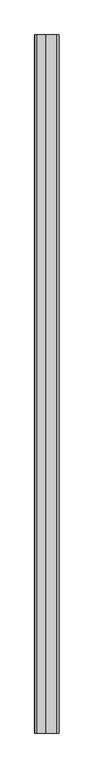
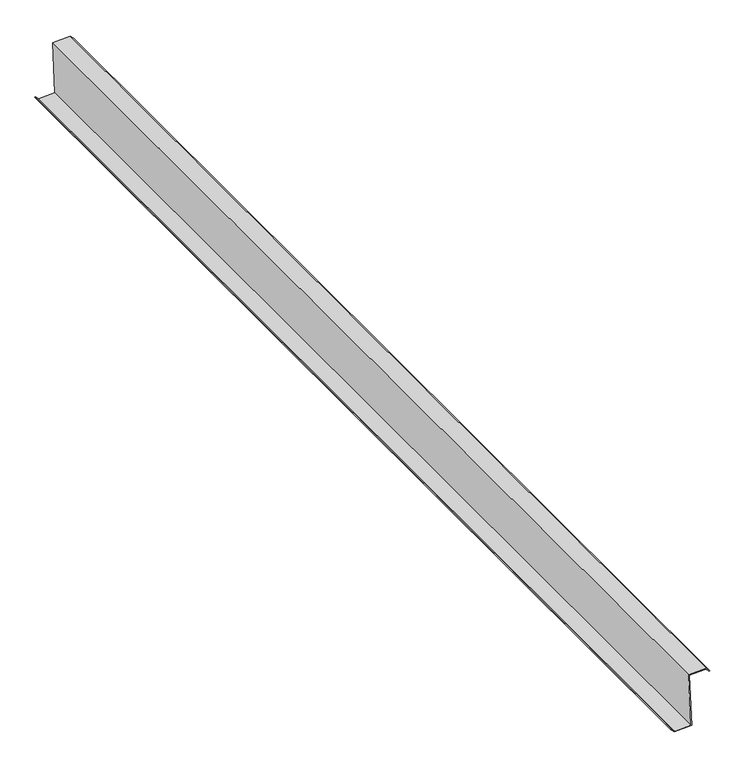
"""IFC4 building model written with IfcOpenShell, lengths in millimetres: proxy geometry, Generic Models 7:Generic Models 1:337419:Generic Models 1:337419 : Generic Models 7:Generic Models 1:337419:3 : Generic Models 7:Generic Models 1:337419:Generic Models 1:337419 : Generic Models 7:Generic Models 1:337419:301336."""

import ifcopenshell
import ifcopenshell.guid

model = None  # the IFC model being written
_history = None  # IfcOwnerHistory: only IFC2X3 demands one
_inside = {}  # id of a spatial element -> (the spatial element, [elements in it])
_under = {}  # id of a project, library or spatial element -> (it, [spatial elements below it])
_declared = {}  # id of a project -> (the project, [libraries it declares])
_typed = {}  # id of a type object -> (the type object, [elements of that type])
_made_of = {}  # id of a material, layer set ... -> (it, [elements and type objects made of it])


def new_model(schema):
    """Start an empty IFC model of exactly this schema.

    Asked for "IFC4X3", IfcOpenShell would pick the latest addendum, in which some entities
    have other attributes; the version numbers below select the first issue.
    IFC2X3 requires an IfcOwnerHistory on every rooted entity: one is made here for all.
    """
    global model, _history
    if schema == "IFC4X3":
        model = ifcopenshell.file(schema_version=(4, 3, 0, 0))
    else:
        model = ifcopenshell.file(schema=schema)
    _inside.clear()
    _under.clear()
    _declared.clear()
    _typed.clear()
    _made_of.clear()
    _history = None
    if model.schema == "IFC2X3":
        org = make("IfcOrganization", Name="unknown")
        user = make(
            "IfcPersonAndOrganization",
            ThePerson=make("IfcPerson", FamilyName="unknown"),
            TheOrganization=org,
        )
        app = make(
            "IfcApplication",
            ApplicationDeveloper=org,
            Version="unknown",
            ApplicationFullName="unknown",
            ApplicationIdentifier="unknown",
        )
        _history = make(
            "IfcOwnerHistory",
            OwningUser=user,
            OwningApplication=app,
            ChangeAction="ADDED",
            CreationDate=0,
        )
    return model


def make(cls, **values):
    """One entity of the class cls with the attributes given. An attribute that is None is left unset."""
    return model.create_entity(
        cls, **{name: value for name, value in values.items() if value is not None}
    )


def rooted(cls, **values):
    """An entity with a GlobalId (a new one), such as an element, a storey or a relation."""
    return make(cls, GlobalId=ifcopenshell.guid.new(), OwnerHistory=_history, **values)


def si_unit(unit_type, name, prefix=None):
    """IfcSIUnit, for example si_unit("LENGTHUNIT", "METRE", prefix="MILLI")."""
    return make("IfcSIUnit", UnitType=unit_type, Prefix=prefix, Name=name)


def assignment(units):
    """IfcUnitAssignment: the units of a project."""
    return None if units is None else make("IfcUnitAssignment", Units=units)


def point(xyz):
    """IfcCartesianPoint."""
    return None if xyz is None else make("IfcCartesianPoint", Coordinates=xyz)


def direction(xyz):
    """IfcDirection."""
    return None if xyz is None else make("IfcDirection", DirectionRatios=xyz)


def frame(location, z_axis=None, x_axis=None):
    """IfcAxis2Placement3D, a coordinate frame: its origin and axes. An axis left out is left unset."""
    return make(
        "IfcAxis2Placement3D",
        Location=point(location),
        Axis=direction(z_axis),
        RefDirection=direction(x_axis),
    )


def origin():
    """The frame at (0, 0, 0) with its axes left unset."""
    return frame((0.0, 0.0, 0.0))


def place(relative_to, where):
    """IfcLocalPlacement: puts the frame where relative to a parent placement (None: the world)."""
    return make(
        "IfcLocalPlacement", PlacementRelTo=relative_to, RelativePlacement=where
    )


def context(
    kind, dimensions, precision=None, world=None, true_north=None, identifier=None
):
    """IfcGeometricRepresentationContext, for example the 3D "Model" context."""
    return make(
        "IfcGeometricRepresentationContext",
        ContextIdentifier=identifier,
        ContextType=kind,
        CoordinateSpaceDimension=dimensions,
        Precision=precision,
        WorldCoordinateSystem=world,
        TrueNorth=true_north,
    )


def project(units=None, contexts=None):
    """IfcProject with its units and contexts."""
    return rooted(
        "IfcProject",
        Name="project",
        RepresentationContexts=contexts,
        UnitsInContext=assignment(units),
    )


def spatial(cls, under=None, at=None, **own):
    """A site, building, storey or space (cls), placed at a placement, below another one or the project."""
    s = rooted(cls, ObjectPlacement=at, **own)
    if under is not None:
        _under.setdefault(under.id(), (under, []))[1].append(s)
    return s


def polyline(points):
    """IfcPolyline through the points."""
    return make("IfcPolyline", Points=[point(p) for p in points])


def outline(outer, holes=None, kind="AREA"):
    """IfcArbitraryClosedProfileDef: a profile drawn as a closed curve; with holes, ...WithVoids."""
    if holes is None:
        return make("IfcArbitraryClosedProfileDef", ProfileType=kind, OuterCurve=outer)
    return make(
        "IfcArbitraryProfileDefWithVoids",
        ProfileType=kind,
        OuterCurve=outer,
        InnerCurves=holes,
    )


def extrude(swept, where, along, depth):
    """IfcExtrudedAreaSolid: the profile swept, set in the frame where, extruded along a direction by depth."""
    return make(
        "IfcExtrudedAreaSolid",
        SweptArea=swept,
        Position=where,
        ExtrudedDirection=direction(along),
        Depth=depth,
    )


def shape(context_of_items, identifier, shape_type, items):
    """IfcShapeRepresentation: the items that make up one representation, for example the "Body"."""
    return make(
        "IfcShapeRepresentation",
        ContextOfItems=context_of_items,
        RepresentationIdentifier=identifier,
        RepresentationType=shape_type,
        Items=items,
    )


def source(mapping_origin, context_of_items, identifier, shape_type, items):
    """IfcRepresentationMap: a shape defined once, which mapped items show again and again."""
    return make(
        "IfcRepresentationMap",
        MappingOrigin=mapping_origin,
        MappedRepresentation=shape(context_of_items, identifier, shape_type, items),
    )


def transform(
    local_origin,
    x_axis=None,
    y_axis=None,
    z_axis=None,
    scale=None,
    scale2=None,
    scale3=None,
    uniform=True,
):
    """IfcCartesianTransformationOperator3D, or its non-uniform kind. x_axis, y_axis, z_axis: its Axis1, 2, 3."""
    if uniform:
        return make(
            "IfcCartesianTransformationOperator3D",
            Axis1=direction(x_axis),
            Axis2=direction(y_axis),
            LocalOrigin=point(local_origin),
            Scale=scale,
            Axis3=direction(z_axis),
        )
    return make(
        "IfcCartesianTransformationOperator3DnonUniform",
        Axis1=direction(x_axis),
        Axis2=direction(y_axis),
        LocalOrigin=point(local_origin),
        Scale=scale,
        Axis3=direction(z_axis),
        Scale2=scale2,
        Scale3=scale3,
    )


def mapped(mapping_source, mapping_target):
    """IfcMappedItem: shows the shape of a source again, moved by a transform."""
    return make(
        "IfcMappedItem", MappingSource=mapping_source, MappingTarget=mapping_target
    )


def made_of(thing, what):
    """Note that an element or type object is made of a material, layer set ...; save() writes the relation."""
    if what is not None:
        _made_of.setdefault(what.id(), (what, []))[1].append(thing)
    return thing


def element(
    cls,
    number,
    at=None,
    inside=None,
    cuts=None,
    type_object=None,
    material=None,
    context=None,
    identifier="Body",
    shape_type=None,
    held_by="IfcProductDefinitionShape",
    body=None,
    shapes=None,
    **own,
):
    """One element of the class cls, such as IfcWall. Its Tag is "e" and its number.

    at: its placement. inside: the storey or other place that contains it. cuts: it is an
    opening in that element (IfcRelVoidsElement). A single representation is given by context,
    identifier, shape_type and body (its items); several are given by shapes. held_by: the class
    of the entity that holds the representations. save() writes the other relations.
    """
    e = rooted(cls, Tag="e%d" % number, ObjectPlacement=at, **own)
    if body is not None:
        shapes = [shape(context, identifier, shape_type, body)]
    if shapes is not None:
        e.Representation = make(held_by, Representations=shapes)
    if inside is not None:
        _inside.setdefault(inside.id(), (inside, []))[1].append(e)
    if cuts is not None:
        rooted(
            "IfcRelVoidsElement", RelatingBuildingElement=cuts, RelatedOpeningElement=e
        )
    if type_object is not None:
        _typed.setdefault(type_object.id(), (type_object, []))[1].append(e)
    return made_of(e, material)


def aggregate(whole, parts):
    """IfcRelAggregates: a whole, such as a stair, and the parts it consists of."""
    return rooted("IfcRelAggregates", RelatingObject=whole, RelatedObjects=parts)


def save(model, path):
    """Write the relations noted so far, then the file.

    IfcRelAggregates (storeys below a building ...), IfcRelContainedInSpatialStructure (elements
    in a storey), IfcRelDefinesByType, IfcRelAssociatesMaterial and IfcRelDeclares: one each for
    every whole, place, type object, material and project.
    """
    for whole, parts in _under.values():
        aggregate(whole, parts)
    for where, things in _inside.values():
        rooted(
            "IfcRelContainedInSpatialStructure",
            RelatedElements=things,
            RelatingStructure=where,
        )
    for kind, things in _typed.values():
        rooted("IfcRelDefinesByType", RelatedObjects=things, RelatingType=kind)
    for what, things in _made_of.values():
        rooted("IfcRelAssociatesMaterial", RelatedObjects=things, RelatingMaterial=what)
    for by, libraries in _declared.values():
        rooted("IfcRelDeclares", RelatingContext=by, RelatedDefinitions=libraries)
    model.write(path)


def generic_models_a7836b3d(model_context):
    return source(origin(), model_context, "Body", "SweptSolid", [
        extrude(outline(polyline([(4456.3413342, 578942.785242), (4656.5894581, 578934.4415702), (4659.1212395, 578995.2043241), (4645.8278437, 579007.3368836), (4647.8801617, 579009.2250162), (4661.9508868, 578996.3830072), (4659.2495198, 578931.5501987), (4459.0013959, 578939.8938706), (4456.4696145, 578879.1311166), (4469.5834853, 578867.1624053), (4467.5311672, 578865.2742727), (4453.6399672, 578877.9524336), (4456.3413342, 578942.785242)])), frame((0.0, -578797.4913841, 0.0), z_axis=(0.0, 1.0, 0.0), x_axis=(0.0, 0.0, 1.0)), (0.0, 0.0, 1.0), 4094.7624605),
    ])


if __name__ == "__main__":
    model = new_model("IFC4")
    model_context = context("Model", 3, world=origin())
    ifc_project = project(units=[si_unit("LENGTHUNIT", "METRE", prefix="MILLI")], contexts=[model_context])
    site = spatial("IfcSite", under=ifc_project)
    building = spatial("IfcBuilding", under=site)
    placement = place(None, origin())
    generic_models_shape = generic_models_a7836b3d(model_context)
    element("IfcBuildingElementProxy", 1, Name="Generic Models 7:Generic Models 1:337419:Generic Models 1:337419 : Generic Models 7:Generic Models 1:337419:3 : Generic Models 7:Generic Models 1:337419:Generic Models 1:337419 : Generic Models 7:Generic Models 1:337419:301336", ObjectType="Generic Models 7:Generic Models 1:337419:Generic Models 1:337419 : Generic Models 7:Generic Models 1:337419:3 : Generic Models 7:Generic Models 1:337419:Generic Models 1:337419 : Generic Models 7:Generic Models 1:337419:301336", at=placement, inside=building, context=model_context, shape_type="MappedRepresentation", body=[
        mapped(generic_models_shape, transform((0.0, 0.0, 0.0), x_axis=(1.0, 0.0, 0.0), y_axis=(0.0, 1.0, 0.0), z_axis=(0.0, 0.0, 1.0))),
    ])
    save(model, "model.ifc")

# Revit data of these elements
# Type "Generic Models 7:Generic Models 1:337419:Generic Models 1:337419 : Generic Models 7:Generic Models 1:337419:3 : Generic Models 7:Generic Models 1:337419:Generic Models 1:337419 : Generic Models 7:Generic Models 1:337419:301336"
#   NameOverride = "Generic Models 7:Generic Models 1:337419:Generic Models 1:337419 : Generic Models 7:Generic Models 1:337419:301336"
#   ObjectTypeOverride = "Generic Models 1:337419 : Generic Models 7:Generic Models 1:337419"
#   Reference = "Generic Models 1"
#   Tag = "301336"
# Element 1 (IfcBuildingElementProxy, "Generic Models 7:Generic Models 1:337419:Generic Models 1:337419 : Generic Models 7:Generic Models 1:337419:3 : Generic Models 7:Generic Models 1:337419:Generic Models 1:337419 : Generic Models 7:Generic Models 1:337419:301336")
#   Materials on its faces: "'ZEE' SECTION (8.0x3.5Z - SEE STRUCT. DWGS)"
# Materials
#   "'ZEE' SECTION (8.0x3.5Z - SEE STRUCT. DWGS)": class "Unassigned", colour RGB 210 209 208, transparency 0, Keynote = "M05121300.02", Cost = 0
